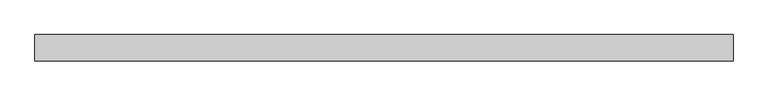
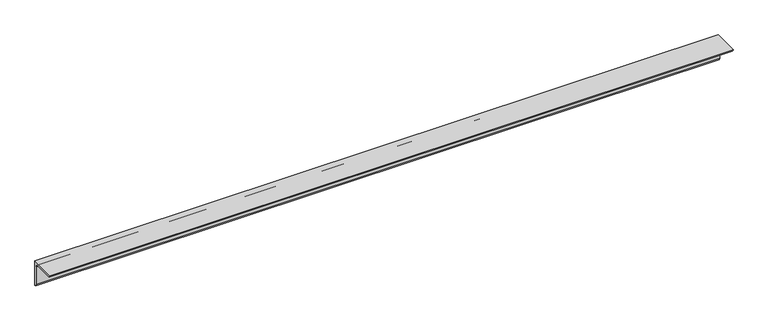
"""IFC4 building model written with IfcOpenShell, lengths in millimetres: member geometry, 0912_Steel Framing_L-KSD3502 : H_SB_AR_S03_L-130x130x12_HBR3."""

from ifc_helpers import new_model, si_unit, point, frame, frame_2d, origin, place, context, project, spatial, polyline, circle_curve, trimmed, segment, composite_curve, outline, extrude, source, transform, mapped, element, save


def member_336a097f(model_context):
    return source(origin(), model_context, "Body", "SweptSolid", [
        extrude(outline(composite_curve([segment(polyline([(36.4, 36.4), (36.4, -93.6)]), True, "CONTINUOUS"), segment(trimmed(circle_curve(frame_2d((36.4, -81.6)), 12.0), [point((36.4, -93.6))], [point((24.4, -81.6))], False, "CARTESIAN"), True, "CONTINUOUS"), segment(polyline([(24.4, -81.6), (24.4, 12.4)]), True, "CONTINUOUS"), segment(trimmed(circle_curve(frame_2d((12.4, 12.4)), 12.0), [point((24.4, 12.4))], [point((12.4, 24.4))], True, "CARTESIAN"), True, "CONTINUOUS"), segment(polyline([(12.4, 24.4), (-81.6, 24.4)]), True, "CONTINUOUS"), segment(trimmed(circle_curve(frame_2d((-81.6, 36.4)), 12.0), [point((-81.6, 24.4))], [point((-93.6, 36.4))], False, "CARTESIAN"), True, "CONTINUOUS"), segment(polyline([(-93.6, 36.4), (36.4, 36.4)]), True, "CONTINUOUS")], self_intersect=False)), frame((-1734.7763172, 0.0, 0.0), z_axis=(1.0, 0.0, 0.0), x_axis=(0.0, 1.0, 0.0)), (0.0, 0.0, 1.0), 3433.9208324),
    ])


if __name__ == "__main__":
    model = new_model("IFC4")
    model_context = context("Model", 3, world=origin())
    ifc_project = project(units=[si_unit("LENGTHUNIT", "METRE", prefix="MILLI")], contexts=[model_context])
    site = spatial("IfcSite", under=ifc_project)
    building = spatial("IfcBuilding", under=site)
    placement = place(None, origin())
    member_shape = member_336a097f(model_context)
    element("IfcMember", 1, ObjectType="0912_Steel Framing_L-KSD3502 : H_SB_AR_S03_L-130x130x12_HBR3", at=placement, inside=building, context=model_context, shape_type="MappedRepresentation", body=[
        mapped(member_shape, transform((0.0, 0.0, 0.0), x_axis=(1.0, 0.0, 0.0), y_axis=(0.0, 1.0, 0.0), z_axis=(0.0, 0.0, 1.0))),
    ])
    save(model, "model.ifc")

# Revit data of these elements
# Type "0912_Steel Framing_L-KSD3502 : H_SB_AR_S03_L-130x130x12_HBR3"
#   k = 25 mm
#   Perimeter = 0.52 m²/m
#   Nominal Weight = 23.40 kgf/m
#   Length [instance default] = 1000 mm
#   b = 130 mm
#   d = 130 mm
#   t = 12 mm
#   x = 36.4 mm
#   y = 36.4 mm
#   A = 2976.00 m²
#   Structural Material [instance default] = Steel, 45-345
# Element 1 (IfcMember, "0912_Steel Framing_L-KSD3502 : H_SB_AR_S03_L-130x130x12_HBR3")
#   Materials on its faces: "Steel, 45-345"
# Materials
#   "Steel, 45-345": class "Metal", colour RGB 189 187 185, transparency 0, Description = "Steel 345 MPa", Cost = 0
